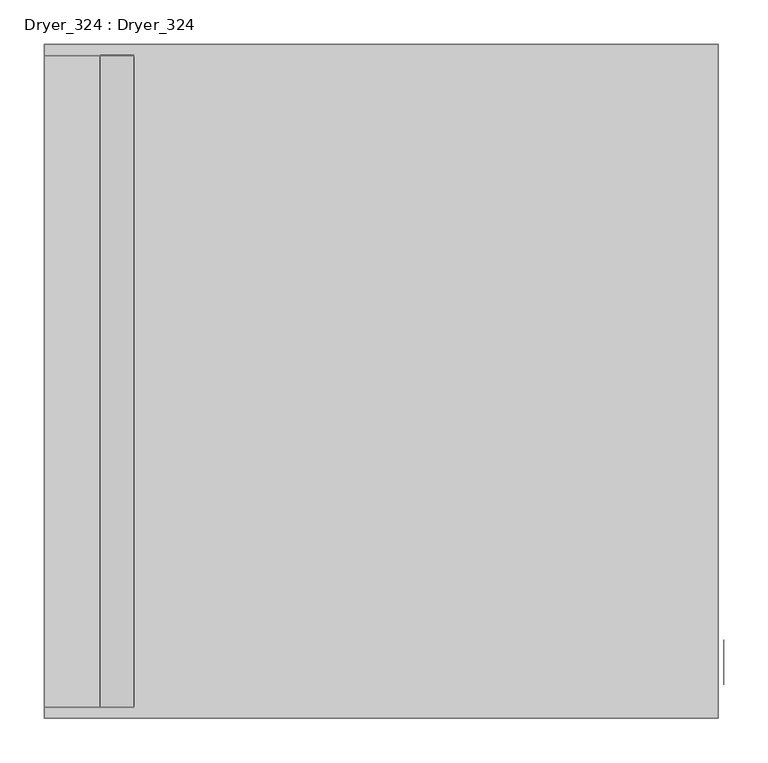
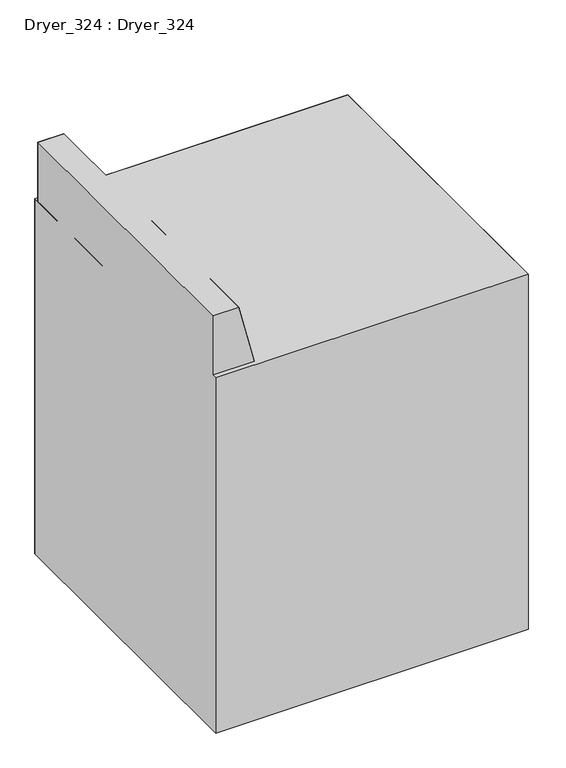
"""IFC4 building model written with IfcOpenShell, lengths in millimetres: proxy geometry, Dryer_324 : Dryer_324."""

from ifc_helpers import new_model, si_unit, origin, place, context, project, spatial, triangles, source, transform, mapped, element, save


def dryer_324_dryer_324_45d75fdb(model_context):
    return source(origin(), model_context, "Body", "Tessellation", [
        triangles([(762.0, 749.2999758, 825.4999758), (762.0, 762.0000727, 838.2), (762.0, 12.7000231, 825.4999758), (762.0, 2.44e-05, 838.2), (762.0, 749.2999758, 292.0999758), (762.0, 761.9999273, 279.3999697), (762.0, 12.6999765, 292.0999939), (762.0, -2.44e-05, 279.4000061)], [[1, 2, 3], [4, 3, 2], [5, 6, 2], [2, 1, 5], [7, 8, 5], [6, 5, 8], [3, 4, 8], [8, 7, 3]], closed=False),
        triangles([(768.3499758, 38.1000045, 647.7), (768.3499758, 38.0999932, 495.3), (768.3499758, 88.9000061, 647.7), (768.3499758, 88.899997, 495.3)], [[1, 2, 3], [4, 3, 2]], closed=False),
        triangles([(762.0, 762.0, 279.3999697), (762.0, -2.22e-05, 279.4000061), (762.0, 761.9999273, -3.33e-05), (762.0, -4.66e-05, 3.33e-05), (0.0, 3.33e-05, 914.4), (0.0, 762.0000727, 914.4), (0.0, 761.9999273, -3.33e-05), (0.0, -4.66e-05, 3.33e-05), (0.0, 749.3000484, 1066.8), (63.4999985, 749.3000484, 1066.8), (0.0, 749.3000484, 914.4), (101.600003, 749.3000484, 914.4), (0.0, 12.7000469, 1066.8), (63.4999985, 12.7000469, 1066.8), (0.0, 12.7000333, 914.4), (101.600003, 12.7000333, 914.4), (762.0, 762.0000727, 914.4), (762.0, 3.33e-05, 914.4), (762.0, 762.0000727, 838.2), (762.0, 2.66e-05, 838.2), (762.0, 749.3000484, 825.4999758), (762.0, 12.7000254, 825.4999758), (762.0, 749.2999758, 292.0999758), (762.0, 12.6999788, 292.0999939)], [[1, 2, 3], [4, 3, 2], [5, 6, 7], [7, 8, 5], [9, 10, 11], [12, 11, 10], [13, 14, 10], [10, 9, 13], [15, 16, 13], [14, 13, 16], [10, 14, 12], [16, 12, 14], [6, 17, 7], [3, 7, 17], [5, 18, 17], [17, 6, 5], [8, 4, 18], [18, 5, 8], [13, 9, 11], [11, 15, 13], [17, 18, 19], [20, 19, 18], [21, 22, 23], [24, 23, 22]], closed=False),
    ])


if __name__ == "__main__":
    model = new_model("IFC4")
    model_context = context("Model", 3, world=origin())
    ifc_project = project(units=[si_unit("LENGTHUNIT", "METRE", prefix="MILLI")], contexts=[model_context])
    site = spatial("IfcSite", under=ifc_project)
    building = spatial("IfcBuilding", under=site)
    placement = place(None, origin())
    dryer_324_dryer_324_shape = dryer_324_dryer_324_45d75fdb(model_context)
    element("IfcBuildingElementProxy", 1, Name="Dryer_324 : Dryer_324", ObjectType="Dryer_324 : Dryer_324", at=placement, inside=building, context=model_context, shape_type="MappedRepresentation", body=[
        mapped(dryer_324_dryer_324_shape, transform((0.0, 0.0, 0.0), x_axis=(1.0, 0.0, 0.0), y_axis=(0.0, 1.0, 0.0), z_axis=(0.0, 0.0, 1.0))),
    ])
    save(model, "model.ifc")

# Revit data of these elements
# Type "Dryer_324 : Dryer_324"
#   Default Elevation = 0
